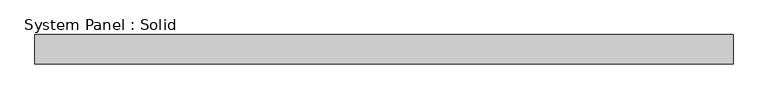
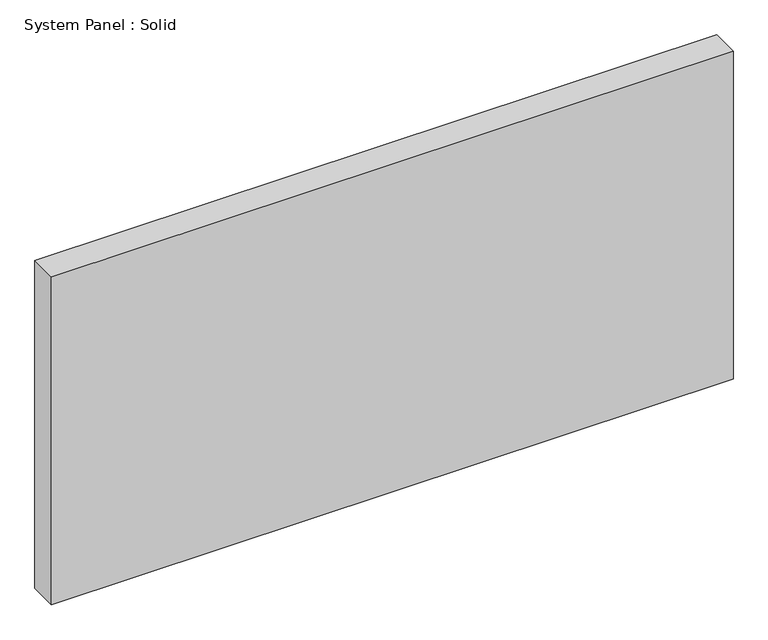
"""IFC4 building model written with IfcOpenShell, lengths in millimetres: plate geometry, System Panel : Solid."""

import ifcopenshell
import ifcopenshell.guid

model = None  # the IFC model being written
_history = None  # IfcOwnerHistory: only IFC2X3 demands one
_inside = {}  # id of a spatial element -> (the spatial element, [elements in it])
_under = {}  # id of a project, library or spatial element -> (it, [spatial elements below it])
_declared = {}  # id of a project -> (the project, [libraries it declares])
_typed = {}  # id of a type object -> (the type object, [elements of that type])
_made_of = {}  # id of a material, layer set ... -> (it, [elements and type objects made of it])


def new_model(schema):
    """Start an empty IFC model of exactly this schema.

    Asked for "IFC4X3", IfcOpenShell would pick the latest addendum, in which some entities
    have other attributes; the version numbers below select the first issue.
    IFC2X3 requires an IfcOwnerHistory on every rooted entity: one is made here for all.
    """
    global model, _history
    if schema == "IFC4X3":
        model = ifcopenshell.file(schema_version=(4, 3, 0, 0))
    else:
        model = ifcopenshell.file(schema=schema)
    _inside.clear()
    _under.clear()
    _declared.clear()
    _typed.clear()
    _made_of.clear()
    _history = None
    if model.schema == "IFC2X3":
        org = make("IfcOrganization", Name="unknown")
        user = make(
            "IfcPersonAndOrganization",
            ThePerson=make("IfcPerson", FamilyName="unknown"),
            TheOrganization=org,
        )
        app = make(
            "IfcApplication",
            ApplicationDeveloper=org,
            Version="unknown",
            ApplicationFullName="unknown",
            ApplicationIdentifier="unknown",
        )
        _history = make(
            "IfcOwnerHistory",
            OwningUser=user,
            OwningApplication=app,
            ChangeAction="ADDED",
            CreationDate=0,
        )
    return model


def make(cls, **values):
    """One entity of the class cls with the attributes given. An attribute that is None is left unset."""
    return model.create_entity(
        cls, **{name: value for name, value in values.items() if value is not None}
    )


def rooted(cls, **values):
    """An entity with a GlobalId (a new one), such as an element, a storey or a relation."""
    return make(cls, GlobalId=ifcopenshell.guid.new(), OwnerHistory=_history, **values)


def si_unit(unit_type, name, prefix=None):
    """IfcSIUnit, for example si_unit("LENGTHUNIT", "METRE", prefix="MILLI")."""
    return make("IfcSIUnit", UnitType=unit_type, Prefix=prefix, Name=name)


def assignment(units):
    """IfcUnitAssignment: the units of a project."""
    return None if units is None else make("IfcUnitAssignment", Units=units)


def point(xyz):
    """IfcCartesianPoint."""
    return None if xyz is None else make("IfcCartesianPoint", Coordinates=xyz)


def direction(xyz):
    """IfcDirection."""
    return None if xyz is None else make("IfcDirection", DirectionRatios=xyz)


def frame(location, z_axis=None, x_axis=None):
    """IfcAxis2Placement3D, a coordinate frame: its origin and axes. An axis left out is left unset."""
    return make(
        "IfcAxis2Placement3D",
        Location=point(location),
        Axis=direction(z_axis),
        RefDirection=direction(x_axis),
    )


def origin():
    """The frame at (0, 0, 0) with its axes left unset."""
    return frame((0.0, 0.0, 0.0))


def origin_with_axes():
    """The frame at (0, 0, 0) with the z axis (0, 0, 1) and the x axis (1, 0, 0) written out."""
    return frame((0.0, 0.0, 0.0), z_axis=(0.0, 0.0, 1.0), x_axis=(1.0, 0.0, 0.0))


def place(relative_to, where):
    """IfcLocalPlacement: puts the frame where relative to a parent placement (None: the world)."""
    return make(
        "IfcLocalPlacement", PlacementRelTo=relative_to, RelativePlacement=where
    )


def context(
    kind, dimensions, precision=None, world=None, true_north=None, identifier=None
):
    """IfcGeometricRepresentationContext, for example the 3D "Model" context."""
    return make(
        "IfcGeometricRepresentationContext",
        ContextIdentifier=identifier,
        ContextType=kind,
        CoordinateSpaceDimension=dimensions,
        Precision=precision,
        WorldCoordinateSystem=world,
        TrueNorth=true_north,
    )


def project(units=None, contexts=None):
    """IfcProject with its units and contexts."""
    return rooted(
        "IfcProject",
        Name="project",
        RepresentationContexts=contexts,
        UnitsInContext=assignment(units),
    )


def spatial(cls, under=None, at=None, **own):
    """A site, building, storey or space (cls), placed at a placement, below another one or the project."""
    s = rooted(cls, ObjectPlacement=at, **own)
    if under is not None:
        _under.setdefault(under.id(), (under, []))[1].append(s)
    return s


def polyline(points):
    """IfcPolyline through the points."""
    return make("IfcPolyline", Points=[point(p) for p in points])


def outline(outer, holes=None, kind="AREA"):
    """IfcArbitraryClosedProfileDef: a profile drawn as a closed curve; with holes, ...WithVoids."""
    if holes is None:
        return make("IfcArbitraryClosedProfileDef", ProfileType=kind, OuterCurve=outer)
    return make(
        "IfcArbitraryProfileDefWithVoids",
        ProfileType=kind,
        OuterCurve=outer,
        InnerCurves=holes,
    )


def extrude(swept, where, along, depth):
    """IfcExtrudedAreaSolid: the profile swept, set in the frame where, extruded along a direction by depth."""
    return make(
        "IfcExtrudedAreaSolid",
        SweptArea=swept,
        Position=where,
        ExtrudedDirection=direction(along),
        Depth=depth,
    )


def shape(context_of_items, identifier, shape_type, items):
    """IfcShapeRepresentation: the items that make up one representation, for example the "Body"."""
    return make(
        "IfcShapeRepresentation",
        ContextOfItems=context_of_items,
        RepresentationIdentifier=identifier,
        RepresentationType=shape_type,
        Items=items,
    )


def source(mapping_origin, context_of_items, identifier, shape_type, items):
    """IfcRepresentationMap: a shape defined once, which mapped items show again and again."""
    return make(
        "IfcRepresentationMap",
        MappingOrigin=mapping_origin,
        MappedRepresentation=shape(context_of_items, identifier, shape_type, items),
    )


def transform(
    local_origin,
    x_axis=None,
    y_axis=None,
    z_axis=None,
    scale=None,
    scale2=None,
    scale3=None,
    uniform=True,
):
    """IfcCartesianTransformationOperator3D, or its non-uniform kind. x_axis, y_axis, z_axis: its Axis1, 2, 3."""
    if uniform:
        return make(
            "IfcCartesianTransformationOperator3D",
            Axis1=direction(x_axis),
            Axis2=direction(y_axis),
            LocalOrigin=point(local_origin),
            Scale=scale,
            Axis3=direction(z_axis),
        )
    return make(
        "IfcCartesianTransformationOperator3DnonUniform",
        Axis1=direction(x_axis),
        Axis2=direction(y_axis),
        LocalOrigin=point(local_origin),
        Scale=scale,
        Axis3=direction(z_axis),
        Scale2=scale2,
        Scale3=scale3,
    )


def mapped(mapping_source, mapping_target):
    """IfcMappedItem: shows the shape of a source again, moved by a transform."""
    return make(
        "IfcMappedItem", MappingSource=mapping_source, MappingTarget=mapping_target
    )


def made_of(thing, what):
    """Note that an element or type object is made of a material, layer set ...; save() writes the relation."""
    if what is not None:
        _made_of.setdefault(what.id(), (what, []))[1].append(thing)
    return thing


def element(
    cls,
    number,
    at=None,
    inside=None,
    cuts=None,
    type_object=None,
    material=None,
    context=None,
    identifier="Body",
    shape_type=None,
    held_by="IfcProductDefinitionShape",
    body=None,
    shapes=None,
    **own,
):
    """One element of the class cls, such as IfcWall. Its Tag is "e" and its number.

    at: its placement. inside: the storey or other place that contains it. cuts: it is an
    opening in that element (IfcRelVoidsElement). A single representation is given by context,
    identifier, shape_type and body (its items); several are given by shapes. held_by: the class
    of the entity that holds the representations. save() writes the other relations.
    """
    e = rooted(cls, Tag="e%d" % number, ObjectPlacement=at, **own)
    if body is not None:
        shapes = [shape(context, identifier, shape_type, body)]
    if shapes is not None:
        e.Representation = make(held_by, Representations=shapes)
    if inside is not None:
        _inside.setdefault(inside.id(), (inside, []))[1].append(e)
    if cuts is not None:
        rooted(
            "IfcRelVoidsElement", RelatingBuildingElement=cuts, RelatedOpeningElement=e
        )
    if type_object is not None:
        _typed.setdefault(type_object.id(), (type_object, []))[1].append(e)
    return made_of(e, material)


def aggregate(whole, parts):
    """IfcRelAggregates: a whole, such as a stair, and the parts it consists of."""
    return rooted("IfcRelAggregates", RelatingObject=whole, RelatedObjects=parts)


def save(model, path):
    """Write the relations noted so far, then the file.

    IfcRelAggregates (storeys below a building ...), IfcRelContainedInSpatialStructure (elements
    in a storey), IfcRelDefinesByType, IfcRelAssociatesMaterial and IfcRelDeclares: one each for
    every whole, place, type object, material and project.
    """
    for whole, parts in _under.values():
        aggregate(whole, parts)
    for where, things in _inside.values():
        rooted(
            "IfcRelContainedInSpatialStructure",
            RelatedElements=things,
            RelatingStructure=where,
        )
    for kind, things in _typed.values():
        rooted("IfcRelDefinesByType", RelatedObjects=things, RelatingType=kind)
    for what, things in _made_of.values():
        rooted("IfcRelAssociatesMaterial", RelatedObjects=things, RelatingMaterial=what)
    for by, libraries in _declared.values():
        rooted("IfcRelDeclares", RelatingContext=by, RelatedDefinitions=libraries)
    model.write(path)


def system_panel_solid_53db45a5(model_context):
    return source(origin(), model_context, "Body", "SweptSolid", [
        extrude(outline(polyline([(712.5, -49.5), (-712.5, -49.5), (-712.5, 10.5), (712.5, 10.5), (712.5, -49.5)])), origin_with_axes(), (0.0, 0.0, 1.0), 725.0),
    ])


if __name__ == "__main__":
    model = new_model("IFC4")
    model_context = context("Model", 3, world=origin())
    ifc_project = project(units=[si_unit("LENGTHUNIT", "METRE", prefix="MILLI")], contexts=[model_context])
    site = spatial("IfcSite", under=ifc_project)
    building = spatial("IfcBuilding", under=site)
    placement = place(None, origin())
    system_panel_solid_shape = system_panel_solid_53db45a5(model_context)
    element("IfcPlate", 1, ObjectType="System Panel : Solid", at=placement, inside=building, context=model_context, shape_type="MappedRepresentation", body=[
        mapped(system_panel_solid_shape, transform((0.0, 0.0, 0.0), x_axis=(1.0, 0.0, 0.0), y_axis=(0.0, 1.0, 0.0), z_axis=(0.0, 0.0, 1.0))),
    ])
    save(model, "model.ifc")

# Revit data of these elements
# Type "System Panel : Solid"
#   Keynote = "H11"
#   Construction Type Id = "MDOOR"
#   Analytic Construction = "Metal"
#   Visual Light Transmittance = 0
#   Solar Heat Gain Coefficient = 0
#   Heat Transfer Coefficient (U) = 3.7021 W/(m²·K)
# Element 1 (IfcPlate, "System Panel : Solid")
#   Materials on its faces: "Default"
# Materials
#   "Default": class "Miscellaneous", colour RGB 127 127 127, transparency 0, Comments = "Rendering appearance not upgraded ", Cost = 0
